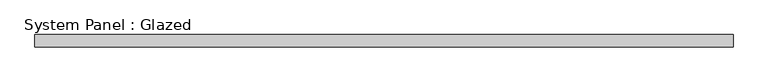
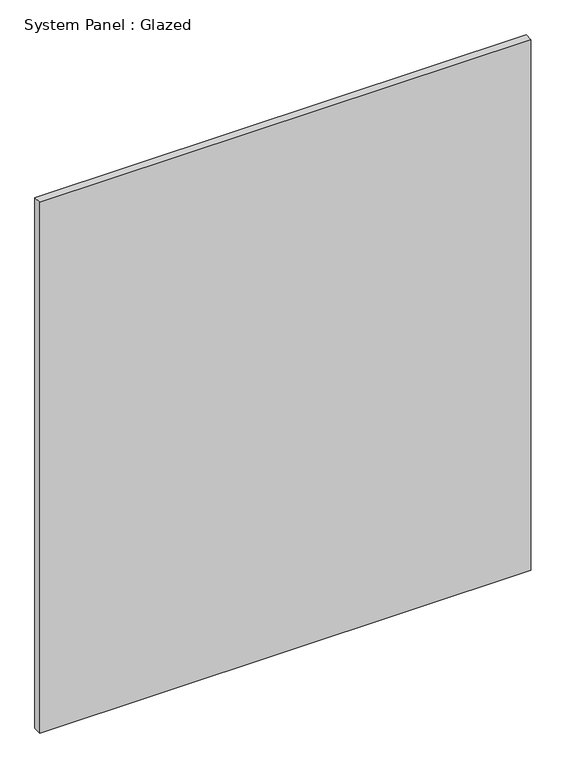
"""IFC4 building model written with IfcOpenShell, lengths in millimetres: plate geometry, System Panel : Glazed."""

import ifcopenshell
import ifcopenshell.guid

model = None  # the IFC model being written
_history = None  # IfcOwnerHistory: only IFC2X3 demands one
_inside = {}  # id of a spatial element -> (the spatial element, [elements in it])
_under = {}  # id of a project, library or spatial element -> (it, [spatial elements below it])
_declared = {}  # id of a project -> (the project, [libraries it declares])
_typed = {}  # id of a type object -> (the type object, [elements of that type])
_made_of = {}  # id of a material, layer set ... -> (it, [elements and type objects made of it])


def new_model(schema):
    """Start an empty IFC model of exactly this schema.

    Asked for "IFC4X3", IfcOpenShell would pick the latest addendum, in which some entities
    have other attributes; the version numbers below select the first issue.
    IFC2X3 requires an IfcOwnerHistory on every rooted entity: one is made here for all.
    """
    global model, _history
    if schema == "IFC4X3":
        model = ifcopenshell.file(schema_version=(4, 3, 0, 0))
    else:
        model = ifcopenshell.file(schema=schema)
    _inside.clear()
    _under.clear()
    _declared.clear()
    _typed.clear()
    _made_of.clear()
    _history = None
    if model.schema == "IFC2X3":
        org = make("IfcOrganization", Name="unknown")
        user = make(
            "IfcPersonAndOrganization",
            ThePerson=make("IfcPerson", FamilyName="unknown"),
            TheOrganization=org,
        )
        app = make(
            "IfcApplication",
            ApplicationDeveloper=org,
            Version="unknown",
            ApplicationFullName="unknown",
            ApplicationIdentifier="unknown",
        )
        _history = make(
            "IfcOwnerHistory",
            OwningUser=user,
            OwningApplication=app,
            ChangeAction="ADDED",
            CreationDate=0,
        )
    return model


def make(cls, **values):
    """One entity of the class cls with the attributes given. An attribute that is None is left unset."""
    return model.create_entity(
        cls, **{name: value for name, value in values.items() if value is not None}
    )


def rooted(cls, **values):
    """An entity with a GlobalId (a new one), such as an element, a storey or a relation."""
    return make(cls, GlobalId=ifcopenshell.guid.new(), OwnerHistory=_history, **values)


def si_unit(unit_type, name, prefix=None):
    """IfcSIUnit, for example si_unit("LENGTHUNIT", "METRE", prefix="MILLI")."""
    return make("IfcSIUnit", UnitType=unit_type, Prefix=prefix, Name=name)


def assignment(units):
    """IfcUnitAssignment: the units of a project."""
    return None if units is None else make("IfcUnitAssignment", Units=units)


def point(xyz):
    """IfcCartesianPoint."""
    return None if xyz is None else make("IfcCartesianPoint", Coordinates=xyz)


def direction(xyz):
    """IfcDirection."""
    return None if xyz is None else make("IfcDirection", DirectionRatios=xyz)


def frame(location, z_axis=None, x_axis=None):
    """IfcAxis2Placement3D, a coordinate frame: its origin and axes. An axis left out is left unset."""
    return make(
        "IfcAxis2Placement3D",
        Location=point(location),
        Axis=direction(z_axis),
        RefDirection=direction(x_axis),
    )


def origin():
    """The frame at (0, 0, 0) with its axes left unset."""
    return frame((0.0, 0.0, 0.0))


def origin_with_axes():
    """The frame at (0, 0, 0) with the z axis (0, 0, 1) and the x axis (1, 0, 0) written out."""
    return frame((0.0, 0.0, 0.0), z_axis=(0.0, 0.0, 1.0), x_axis=(1.0, 0.0, 0.0))


def place(relative_to, where):
    """IfcLocalPlacement: puts the frame where relative to a parent placement (None: the world)."""
    return make(
        "IfcLocalPlacement", PlacementRelTo=relative_to, RelativePlacement=where
    )


def context(
    kind, dimensions, precision=None, world=None, true_north=None, identifier=None
):
    """IfcGeometricRepresentationContext, for example the 3D "Model" context."""
    return make(
        "IfcGeometricRepresentationContext",
        ContextIdentifier=identifier,
        ContextType=kind,
        CoordinateSpaceDimension=dimensions,
        Precision=precision,
        WorldCoordinateSystem=world,
        TrueNorth=true_north,
    )


def project(units=None, contexts=None):
    """IfcProject with its units and contexts."""
    return rooted(
        "IfcProject",
        Name="project",
        RepresentationContexts=contexts,
        UnitsInContext=assignment(units),
    )


def spatial(cls, under=None, at=None, **own):
    """A site, building, storey or space (cls), placed at a placement, below another one or the project."""
    s = rooted(cls, ObjectPlacement=at, **own)
    if under is not None:
        _under.setdefault(under.id(), (under, []))[1].append(s)
    return s


def polyline(points):
    """IfcPolyline through the points."""
    return make("IfcPolyline", Points=[point(p) for p in points])


def outline(outer, holes=None, kind="AREA"):
    """IfcArbitraryClosedProfileDef: a profile drawn as a closed curve; with holes, ...WithVoids."""
    if holes is None:
        return make("IfcArbitraryClosedProfileDef", ProfileType=kind, OuterCurve=outer)
    return make(
        "IfcArbitraryProfileDefWithVoids",
        ProfileType=kind,
        OuterCurve=outer,
        InnerCurves=holes,
    )


def extrude(swept, where, along, depth):
    """IfcExtrudedAreaSolid: the profile swept, set in the frame where, extruded along a direction by depth."""
    return make(
        "IfcExtrudedAreaSolid",
        SweptArea=swept,
        Position=where,
        ExtrudedDirection=direction(along),
        Depth=depth,
    )


def shape(context_of_items, identifier, shape_type, items):
    """IfcShapeRepresentation: the items that make up one representation, for example the "Body"."""
    return make(
        "IfcShapeRepresentation",
        ContextOfItems=context_of_items,
        RepresentationIdentifier=identifier,
        RepresentationType=shape_type,
        Items=items,
    )


def source(mapping_origin, context_of_items, identifier, shape_type, items):
    """IfcRepresentationMap: a shape defined once, which mapped items show again and again."""
    return make(
        "IfcRepresentationMap",
        MappingOrigin=mapping_origin,
        MappedRepresentation=shape(context_of_items, identifier, shape_type, items),
    )


def transform(
    local_origin,
    x_axis=None,
    y_axis=None,
    z_axis=None,
    scale=None,
    scale2=None,
    scale3=None,
    uniform=True,
):
    """IfcCartesianTransformationOperator3D, or its non-uniform kind. x_axis, y_axis, z_axis: its Axis1, 2, 3."""
    if uniform:
        return make(
            "IfcCartesianTransformationOperator3D",
            Axis1=direction(x_axis),
            Axis2=direction(y_axis),
            LocalOrigin=point(local_origin),
            Scale=scale,
            Axis3=direction(z_axis),
        )
    return make(
        "IfcCartesianTransformationOperator3DnonUniform",
        Axis1=direction(x_axis),
        Axis2=direction(y_axis),
        LocalOrigin=point(local_origin),
        Scale=scale,
        Axis3=direction(z_axis),
        Scale2=scale2,
        Scale3=scale3,
    )


def mapped(mapping_source, mapping_target):
    """IfcMappedItem: shows the shape of a source again, moved by a transform."""
    return make(
        "IfcMappedItem", MappingSource=mapping_source, MappingTarget=mapping_target
    )


def made_of(thing, what):
    """Note that an element or type object is made of a material, layer set ...; save() writes the relation."""
    if what is not None:
        _made_of.setdefault(what.id(), (what, []))[1].append(thing)
    return thing


def element(
    cls,
    number,
    at=None,
    inside=None,
    cuts=None,
    type_object=None,
    material=None,
    context=None,
    identifier="Body",
    shape_type=None,
    held_by="IfcProductDefinitionShape",
    body=None,
    shapes=None,
    **own,
):
    """One element of the class cls, such as IfcWall. Its Tag is "e" and its number.

    at: its placement. inside: the storey or other place that contains it. cuts: it is an
    opening in that element (IfcRelVoidsElement). A single representation is given by context,
    identifier, shape_type and body (its items); several are given by shapes. held_by: the class
    of the entity that holds the representations. save() writes the other relations.
    """
    e = rooted(cls, Tag="e%d" % number, ObjectPlacement=at, **own)
    if body is not None:
        shapes = [shape(context, identifier, shape_type, body)]
    if shapes is not None:
        e.Representation = make(held_by, Representations=shapes)
    if inside is not None:
        _inside.setdefault(inside.id(), (inside, []))[1].append(e)
    if cuts is not None:
        rooted(
            "IfcRelVoidsElement", RelatingBuildingElement=cuts, RelatedOpeningElement=e
        )
    if type_object is not None:
        _typed.setdefault(type_object.id(), (type_object, []))[1].append(e)
    return made_of(e, material)


def aggregate(whole, parts):
    """IfcRelAggregates: a whole, such as a stair, and the parts it consists of."""
    return rooted("IfcRelAggregates", RelatingObject=whole, RelatedObjects=parts)


def save(model, path):
    """Write the relations noted so far, then the file.

    IfcRelAggregates (storeys below a building ...), IfcRelContainedInSpatialStructure (elements
    in a storey), IfcRelDefinesByType, IfcRelAssociatesMaterial and IfcRelDeclares: one each for
    every whole, place, type object, material and project.
    """
    for whole, parts in _under.values():
        aggregate(whole, parts)
    for where, things in _inside.values():
        rooted(
            "IfcRelContainedInSpatialStructure",
            RelatedElements=things,
            RelatingStructure=where,
        )
    for kind, things in _typed.values():
        rooted("IfcRelDefinesByType", RelatedObjects=things, RelatingType=kind)
    for what, things in _made_of.values():
        rooted("IfcRelAssociatesMaterial", RelatedObjects=things, RelatingMaterial=what)
    for by, libraries in _declared.values():
        rooted("IfcRelDeclares", RelatingContext=by, RelatedDefinitions=libraries)
    model.write(path)


def system_panel_glazed_d30dad71(model_context):
    return source(origin(), model_context, "Body", "SweptSolid", [
        extrude(outline(polyline([(718.0084626, 24.5), (-718.0084626, 24.5), (-718.0084626, 49.5), (718.0084626, 49.5), (718.0084626, 24.5)])), origin_with_axes(), (0.0, 0.0, 1.0), 1640.2939092),
    ])


if __name__ == "__main__":
    model = new_model("IFC4")
    model_context = context("Model", 3, world=origin())
    ifc_project = project(units=[si_unit("LENGTHUNIT", "METRE", prefix="MILLI")], contexts=[model_context])
    site = spatial("IfcSite", under=ifc_project)
    building = spatial("IfcBuilding", under=site)
    placement = place(None, origin())
    system_panel_glazed_shape = system_panel_glazed_d30dad71(model_context)
    element("IfcPlate", 1, ObjectType="System Panel : Glazed", at=placement, inside=building, context=model_context, shape_type="MappedRepresentation", body=[
        mapped(system_panel_glazed_shape, transform((0.0, 0.0, 0.0), x_axis=(1.0, 0.0, 0.0), y_axis=(0.0, 1.0, 0.0), z_axis=(0.0, 0.0, 1.0))),
    ])
    save(model, "model.ifc")

# Revit data of these elements
# Element 1 (IfcPlate, "System Panel : Glazed")
#   Materials on its faces: "Glass"
# Materials
#   "Glass": class "Glass", colour RGB 218 227 224, transparency 0.85, Description = "Soda Lime Glass", Cost = 0
